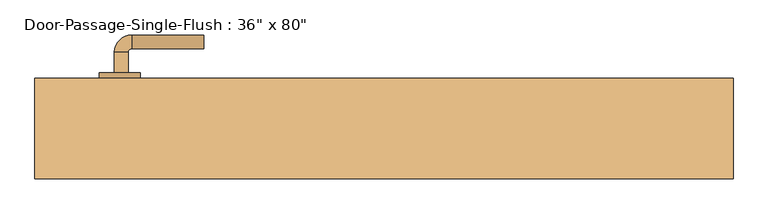
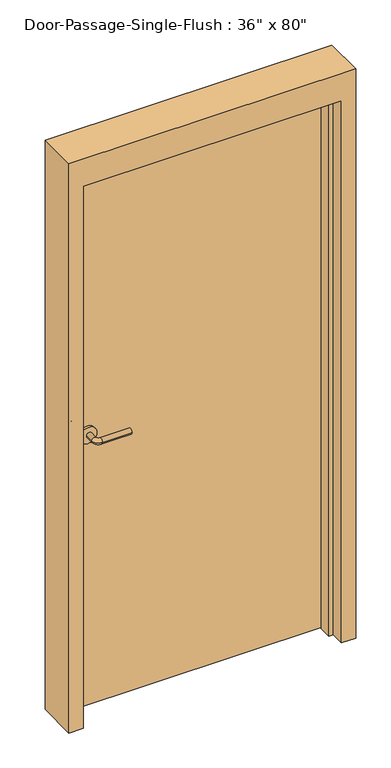
"""IFC4 building model written with IfcOpenShell, lengths in millimetres: door geometry."""

from ifc_helpers import new_model, si_unit, point, frame, frame_2d, origin, origin_with_axes, place, context, project, spatial, polyline, circle_curve, ellipse_curve, trimmed, segment, composite_curve, outline, extrude, faceted_brep, source, transform, mapped, element, save
from ifc_brep_helpers import plane_surface, cylinder_surface, revolved_surface, advanced_brep


def door_3cdf056c(model_context):
    return source(origin(), model_context, "Body", "SolidModel", [
        advanced_brep(
        [(-392.190625, 26.925, 1016.0), (-372.190625, 26.925, 1016.0), (-372.190625, -3.075, 1016.0), (-392.190625, -3.075, 1016.0), (-367.190625, -8.075, 1016.0), (-367.190625, -28.075, 1016.0), (-262.190625, -28.075, 1016.0), (-262.190625, -8.075, 1016.0)],
        [
            (0, 1, circle_curve(frame((-382.190625, 26.925, 1016.0), z_axis=(0.0, 1.0, 0.0), x_axis=(1.0, 0.0, 0.0)), 10.0)),
            (1, 0, circle_curve(frame((-382.190625, 26.925, 1016.0), z_axis=(0.0, 1.0, 0.0), x_axis=(1.0, 0.0, 0.0)), 10.0)),
            (1, 2),
            (2, 3, circle_curve(frame((-382.190625, -3.075, 1016.0), z_axis=(0.0, 1.0, 0.0), x_axis=(1.0, 0.0, 0.0)), 10.0)),
            (3, 0),
            (3, 2, circle_curve(frame((-382.190625, -3.075, 1016.0), z_axis=(0.0, 1.0, 0.0), x_axis=(1.0, 0.0, 0.0)), 10.0)),
            (4, 5, circle_curve(frame((-367.190625, -18.075, 1016.0), z_axis=(-1.0, 0.0, 0.0), x_axis=(0.0, 1.0, 0.0)), 10.0)),
            (5, 3, circle_curve(frame((-367.190625, -3.075, 1016.0), z_axis=(0.0, 0.0, -1.0), x_axis=(-1.0, 0.0, 0.0)), 25.0)),
            (2, 4, circle_curve(frame((-367.190625, -3.075, 1016.0), z_axis=(0.0, 0.0, 1.0), x_axis=(-1.0, 0.0, 0.0)), 5.0)),
            (5, 4, circle_curve(frame((-367.190625, -18.075, 1016.0), z_axis=(-1.0, 0.0, 0.0), x_axis=(0.0, 1.0, 0.0)), 10.0)),
            (6, 7, circle_curve(frame((-262.190625, -18.075, 1016.0), z_axis=(1.0, 0.0, 0.0), x_axis=(0.0, 1.0, 0.0)), 10.0)),
            (7, 6, circle_curve(frame((-262.190625, -18.075, 1016.0), z_axis=(1.0, 0.0, 0.0), x_axis=(0.0, 1.0, 0.0)), 10.0)),
            (4, 7),
            (6, 5),
        ],
        [
            plane_surface(frame((-382.190625, 26.925, 1016.0), z_axis=(0.0, 1.0, 0.0), x_axis=(0.0, 0.0, 1.0))),
            cylinder_surface(frame((-382.190625, 26.925, 1016.0), z_axis=(0.0, 1.0, 0.0), x_axis=(1.0, 0.0, 0.0)), 10.0),
            revolved_surface(trimmed(ellipse_curve(frame((-382.190625, -3.075, 1016.0), z_axis=(0.0, -1.0, 0.0), x_axis=(1.0, 0.0, 0.0)), 10.0, 10.0), [point((-392.190625, -3.075, 1016.0))], [point((-372.190625, -3.075, 1016.0))], True, "CARTESIAN"), (-367.190625, -3.075, 1016.0), (0.0, 0.0, -1.0)),
            revolved_surface(trimmed(ellipse_curve(frame((-382.190625, -3.075, 1016.0), z_axis=(0.0, -1.0, 0.0), x_axis=(1.0, 0.0, 0.0)), 10.0, 10.0), [point((-372.190625, -3.075, 1016.0))], [point((-392.190625, -3.075, 1016.0))], True, "CARTESIAN"), (-367.190625, -3.075, 1016.0), (0.0, 0.0, -1.0)),
            plane_surface(frame((-262.190625, -18.075, 1016.0), z_axis=(1.0, 0.0, 0.0), x_axis=(0.0, 0.0, 1.0))),
            cylinder_surface(frame((-367.190625, -18.075, 1016.0), z_axis=(-1.0, 0.0, 0.0), x_axis=(0.0, 1.0, 0.0)), 10.0),
        ],
        [
            (0, [[1, 2]]),
            (1, [[3, 4, 5, -2]]),
            (1, [[-5, 6, -3, -1]]),
            (2, [[7, 8, -4, 9]]),
            (3, [[10, -9, -6, -8]]),
            (4, [[11, 12]]),
            (5, [[13, -11, 14, -7]]),
            (5, [[-14, -12, -13, -10]]),
        ],
    ),
        extrude(outline(composite_curve([segment(trimmed(circle_curve(frame_2d((1016.0, -384.690625)), 30.0), [point((1016.0, -414.690625))], [point((1016.0, -354.690625))], False, "CARTESIAN"), True, "CONTINUOUS"), segment(trimmed(circle_curve(frame_2d((1016.0, -384.690625)), 30.0), [point((1016.0, -354.690625))], [point((1016.0, -414.690625))], False, "CARTESIAN"), True, "CONTINUOUS")], self_intersect=False)), frame((0.0, 26.925, 0.0), z_axis=(0.0, 1.0, 0.0), x_axis=(0.0, 0.0, 1.0)), (0.0, 0.0, 1.0), 8.0),
        advanced_brep(
        [(-392.190625, 87.375, 1016.0), (-372.190625, 87.375, 1016.0), (-392.190625, 117.375, 1016.0), (-372.190625, 117.375, 1016.0), (-367.190625, 122.375, 1016.0), (-367.190625, 142.375, 1016.0), (-262.190625, 142.375, 1016.0), (-262.190625, 122.375, 1016.0)],
        [
            (0, 1, circle_curve(frame((-382.190625, 87.375, 1016.0), z_axis=(0.0, -1.0, 0.0), x_axis=(1.0, 0.0, 0.0)), 10.0)),
            (1, 0, circle_curve(frame((-382.190625, 87.375, 1016.0), z_axis=(0.0, -1.0, 0.0), x_axis=(1.0, 0.0, 0.0)), 10.0)),
            (0, 2),
            (2, 3, circle_curve(frame((-382.190625, 117.375, 1016.0), z_axis=(0.0, -1.0, 0.0), x_axis=(1.0, 0.0, 0.0)), 10.0)),
            (3, 1),
            (3, 2, circle_curve(frame((-382.190625, 117.375, 1016.0), z_axis=(0.0, -1.0, 0.0), x_axis=(1.0, 0.0, 0.0)), 10.0)),
            (4, 3, circle_curve(frame((-367.190625, 117.375, 1016.0), z_axis=(0.0, 0.0, 1.0), x_axis=(-1.0, 0.0, 0.0)), 5.0)),
            (2, 5, circle_curve(frame((-367.190625, 117.375, 1016.0), z_axis=(0.0, 0.0, -1.0), x_axis=(-1.0, 0.0, 0.0)), 25.0)),
            (5, 4, circle_curve(frame((-367.190625, 132.375, 1016.0), z_axis=(-1.0, 0.0, 0.0), x_axis=(0.0, -1.0, 0.0)), 10.0)),
            (4, 5, circle_curve(frame((-367.190625, 132.375, 1016.0), z_axis=(-1.0, 0.0, 0.0), x_axis=(0.0, -1.0, 0.0)), 10.0)),
            (6, 7, circle_curve(frame((-262.190625, 132.375, 1016.0), z_axis=(1.0, 0.0, 0.0), x_axis=(0.0, -1.0, 0.0)), 10.0)),
            (7, 6, circle_curve(frame((-262.190625, 132.375, 1016.0), z_axis=(1.0, 0.0, 0.0), x_axis=(0.0, -1.0, 0.0)), 10.0)),
            (5, 6),
            (7, 4),
        ],
        [
            plane_surface(frame((-382.190625, 87.375, 1016.0), z_axis=(0.0, -1.0, 0.0), x_axis=(0.0, 0.0, 1.0))),
            cylinder_surface(frame((-382.190625, 87.375, 1016.0), z_axis=(0.0, -1.0, 0.0), x_axis=(1.0, 0.0, 0.0)), 10.0),
            revolved_surface(trimmed(ellipse_curve(frame((-382.190625, 117.375, 1016.0), z_axis=(0.0, -1.0, 0.0), x_axis=(1.0, 0.0, 0.0)), 10.0, 10.0), [point((-392.190625, 117.375, 1016.0))], [point((-372.190625, 117.375, 1016.0))], True, "CARTESIAN"), (-367.190625, 117.375, 1016.0), (0.0, 0.0, -1.0)),
            revolved_surface(trimmed(ellipse_curve(frame((-382.190625, 117.375, 1016.0), z_axis=(0.0, -1.0, 0.0), x_axis=(1.0, 0.0, 0.0)), 10.0, 10.0), [point((-372.190625, 117.375, 1016.0))], [point((-392.190625, 117.375, 1016.0))], True, "CARTESIAN"), (-367.190625, 117.375, 1016.0), (0.0, 0.0, -1.0)),
            plane_surface(frame((-262.190625, 132.375, 1016.0), z_axis=(1.0, 0.0, 0.0), x_axis=(0.0, 0.0, 1.0))),
            cylinder_surface(frame((-367.190625, 132.375, 1016.0), z_axis=(-1.0, 0.0, 0.0), x_axis=(0.0, -1.0, 0.0)), 10.0),
        ],
        [
            (0, [[1, 2]]),
            (1, [[-1, 3, 4, 5]]),
            (1, [[-2, -5, 6, -3]]),
            (2, [[7, -4, 8, 9]]),
            (3, [[-8, -6, -7, 10]]),
            (4, [[11, 12]]),
            (5, [[-9, 13, -12, 14]]),
            (5, [[-10, -14, -11, -13]]),
        ],
    ),
        extrude(outline(composite_curve([segment(trimmed(circle_curve(frame_2d((1016.0, -384.690625)), 30.0), [point((1016.0, -414.690625))], [point((1016.0, -354.690625))], False, "CARTESIAN"), True, "CONTINUOUS"), segment(trimmed(circle_curve(frame_2d((1016.0, -384.690625)), 30.0), [point((1016.0, -354.690625))], [point((1016.0, -414.690625))], False, "CARTESIAN"), True, "CONTINUOUS")], self_intersect=False)), frame((0.0, 79.375, 0.0), z_axis=(0.0, 1.0, 0.0), x_axis=(0.0, 0.0, 1.0)), (0.0, 0.0, 1.0), 8.0),
        faceted_brep([(457.2, 30.1625, 0.0), (457.2, 79.375, 0.0), (508.0, 79.375, 0.0), (508.0, -66.675, 0.0), (457.2, -66.675, 0.0), (457.2, -17.4625, 0.0), (441.325, -17.4625, 0.0), (441.325, 30.1625, 0.0), (457.2, 30.1625, 2032.0), (457.2, 79.375, 2032.0), (-457.2, 79.375, 2032.0), (-457.2, 79.375, 0.0), (-508.0, 79.375, 0.0), (-508.0, 79.375, 2133.6), (508.0, 79.375, 2133.6), (508.0, -66.675, 2133.6), (-508.0, -66.675, 2133.6), (-508.0, -66.675, 0.0), (-457.2, -66.675, 0.0), (-457.2, -66.675, 2032.0), (457.2, -66.675, 2032.0), (457.2, -17.4625, 2032.0), (-457.2, -17.4625, 2032.0), (-457.2, -17.4625, 0.0), (-441.325, -17.4625, 0.0), (-441.325, -17.4625, 2016.125), (441.325, -17.4625, 2016.125), (441.325, 30.1625, 2016.125), (-441.325, 30.1625, 2016.125), (-441.325, 30.1625, 0.0), (-457.2, 30.1625, 0.0), (-457.2, 30.1625, 2032.0)], [[[0, 1, 2, 3, 4, 5, 6, 7]], [[1, 0, 8, 9]], [[2, 1, 9, 10, 11, 12, 13, 14]], [[3, 2, 14, 15]], [[4, 3, 15, 16, 17, 18, 19, 20]], [[5, 4, 20, 21]], [[6, 5, 21, 22, 23, 24, 25, 26]], [[7, 6, 26, 27]], [[0, 7, 27, 28, 29, 30, 31, 8]], [[9, 8, 31, 10]], [[20, 19, 22, 21]], [[26, 25, 28, 27]], [[12, 11, 30, 29, 24, 23, 18, 17]], [[11, 10, 31, 30]], [[13, 12, 17, 16]], [[19, 18, 23, 22]], [[25, 24, 29, 28]], [[15, 14, 13, 16]]]),
        extrude(outline(polyline([(457.2, 34.925), (-457.2, 34.925), (-457.2, 79.375), (457.2, 79.375), (457.2, 34.925)])), origin_with_axes(), (0.0, 0.0, 1.0), 2032.0),
    ])


if __name__ == "__main__":
    model = new_model("IFC4")
    model_context = context("Model", 3, world=origin())
    ifc_project = project(units=[si_unit("LENGTHUNIT", "METRE", prefix="MILLI")], contexts=[model_context])
    site = spatial("IfcSite", under=ifc_project)
    building = spatial("IfcBuilding", under=site)
    placement = place(None, origin())
    door_shape = door_3cdf056c(model_context)
    element("IfcDoor", 1, ObjectType="Door-Passage-Single-Flush : 36\" x 80\"", at=placement, inside=building, context=model_context, shape_type="MappedRepresentation", body=[
        mapped(door_shape, transform((0.0, 0.0, 0.0), x_axis=(1.0, 0.0, 0.0), y_axis=(0.0, 1.0, 0.0), z_axis=(0.0, 0.0, 1.0))),
    ])
    save(model, "model.ifc")

# Revit data of these elements
# Type "Door-Passage-Single-Flush : 36\" x 80\""
#   Type Mark = "16"
#   Assembly Code = "B2030200"
#   Analytic Construction = "Wooden"
#   Thickness = 0' - 1 3/4"
#   Thermal Resistance (R) = 0.455703 (m²·K)/W
#   Swing Angle [instance default] = 90.00°
#   Strike Height = 3' - 4"
#   Rough Width [instance default] = 3' - 4"
#   Rough Height [instance default] = 7' - 0"
#   MF Opening Height [instance default] = 0' - 4"
#   MF Opening Width [instance default] = 0' - 4"
#   Inset Calculate [instance default] = 0' - 4"
#   Masonry Inset [instance default] = 0' - 1"
#   Height = 6' - 8"
#   Width = 3' - 0"
#   Heat Transfer Coefficient (U) = 2.19465 W/(m²·K)
#   Masonry Frame Depth = 0' - 5 3/4"
#   Masonry Frame [instance default] = yes
#   Function = 1
#   Dry Wall Frame [instance default] = no
#   Panel Material = Wood - Birch
#   Frame Material = Metal - Paint Finish - Grey
#   Door Handle Material = Aluminum
#   Visual Light Transmittance = 0
#   Solar Heat Gain Coefficient = 0
#   Wall Closure = (empty or 0)
# Element 1 (IfcDoor, "Door-Passage-Single-Flush : 36\" x 80\"")
#   Inset Calculate = 0' - 2 1/2"
#   Masonry Inset = -0' - 0 1/2"
#   Materials on its faces: "Aluminum", "Metal - Paint Finish - Grey", "Wood - Birch"
# Materials
#   "Wood - Birch": class "Wood", colour RGB 166 116 52, transparency 0, Cost = 0
#   "Metal - Paint Finish - Grey": class "Paint", colour RGB 104 104 104, transparency 0, Cost = 0
#   "Aluminum": class "Metal", colour RGB 247 247 247, transparency 0, Description = "Aluminum 6061", Cost = 0
